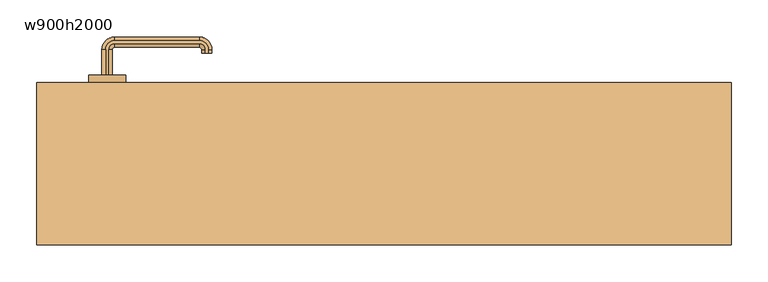
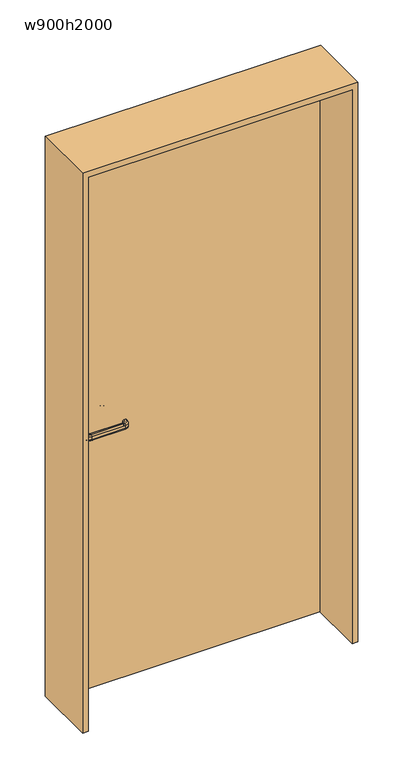
"""IFC4 building model written with IfcOpenShell, lengths in millimetres: door geometry, 片開き : w900h2000."""

from ifc_helpers import new_model, si_unit, point, frame, frame_2d, origin, origin_with_axes, place, context, project, spatial, polyline, circle_curve, ellipse_curve, trimmed, segment, composite_curve, outline, extrude, source, transform, mapped, element, save
from ifc_brep_helpers import plane_surface, cylinder_surface, revolved_surface, advanced_brep


def w900h2000_79a0ba88(model_context):
    return source(origin(), model_context, "Body", "SolidModel", [
        advanced_brep(
        [(-377.0, 120.0, 960.0), (-382.0, 120.0, 955.0), (-382.0, 120.0, 945.0477623), (-377.0, 120.0, 940.0477623), (-373.0, 120.0, 940.0477623), (-368.0, 120.0, 945.0477623), (-368.0, 120.0, 955.0), (-373.0, 120.0, 960.0), (-377.0, 155.0, 960.0), (-382.0, 155.0, 955.0), (-382.0, 155.0, 945.0477623), (-377.0, 155.0, 940.0477623), (-365.0, 167.0, 940.0477623), (-250.0, 167.0, 940.0477623), (-238.0, 155.0, 940.0477623), (-238.0, 150.0, 940.0477623), (-242.0, 150.0, 940.0477623), (-242.0, 155.0, 940.0477623), (-250.0, 163.0, 940.0477623), (-365.0, 163.0, 940.0477623), (-373.0, 155.0, 940.0477623), (-368.0, 155.0, 945.0477623), (-368.0, 155.0, 955.0), (-373.0, 155.0, 960.0), (-365.0, 163.0, 960.0), (-250.0, 163.0, 960.0), (-242.0, 155.0, 960.0), (-242.0, 150.0, 960.0), (-238.0, 150.0, 960.0), (-238.0, 155.0, 960.0), (-250.0, 167.0, 960.0), (-365.0, 167.0, 960.0), (-365.0, 172.0, 955.0), (-365.0, 172.0, 945.0477623), (-365.0, 158.0, 945.0477623), (-365.0, 158.0, 955.0), (-250.0, 172.0, 955.0), (-250.0, 172.0, 945.0477623), (-250.0, 158.0, 945.0477623), (-250.0, 158.0, 955.0), (-233.0, 155.0, 955.0), (-233.0, 155.0, 945.0477623), (-247.0, 155.0, 945.0477623), (-247.0, 155.0, 955.0), (-247.0, 150.0, 955.0), (-247.0, 150.0, 945.0477623), (-233.0, 150.0, 945.0477623), (-233.0, 150.0, 955.0)],
        [
            (0, 1, circle_curve(frame((-377.0, 120.0, 955.0), z_axis=(0.0, -1.0, 0.0), x_axis=(-1.0, 0.0, 0.0)), 5.0)),
            (1, 2),
            (2, 3, circle_curve(frame((-377.0, 120.0, 945.0477623), z_axis=(0.0, -1.0, 0.0), x_axis=(-1.0, 0.0, 0.0)), 5.0)),
            (3, 4),
            (4, 5, circle_curve(frame((-373.0, 120.0, 945.0477623), z_axis=(0.0, -1.0, 0.0), x_axis=(-1.0, 0.0, 0.0)), 5.0)),
            (5, 6),
            (6, 7, circle_curve(frame((-373.0, 120.0, 955.0), z_axis=(0.0, -1.0, 0.0), x_axis=(-1.0, 0.0, 0.0)), 5.0)),
            (7, 0),
            (0, 8),
            (8, 9, circle_curve(frame((-377.0, 155.0, 955.0), z_axis=(0.0, -1.0, 0.0), x_axis=(-1.0, 0.0, 0.0)), 5.0)),
            (9, 1),
            (9, 10),
            (10, 2),
            (10, 11, circle_curve(frame((-377.0, 155.0, 945.0477623), z_axis=(0.0, -1.0, 0.0), x_axis=(-1.0, 0.0, 0.0)), 5.0)),
            (11, 3),
            (11, 12, circle_curve(frame((-365.0, 155.0, 940.0477623), z_axis=(0.0, 0.0, -1.0), x_axis=(-1.0, 0.0, 0.0)), 12.0)),
            (12, 13),
            (13, 14, circle_curve(frame((-250.0, 155.0, 940.0477623), z_axis=(0.0, 0.0, -1.0), x_axis=(0.0, 1.0, 0.0)), 12.0)),
            (14, 15),
            (15, 16),
            (16, 17),
            (17, 18, circle_curve(frame((-250.0, 155.0, 940.0477623), z_axis=(0.0, 0.0, 1.0), x_axis=(0.0, 1.0, 0.0)), 8.0)),
            (18, 19),
            (19, 20, circle_curve(frame((-365.0, 155.0, 940.0477623), z_axis=(0.0, 0.0, 1.0), x_axis=(-1.0, 0.0, 0.0)), 8.0)),
            (20, 4),
            (20, 21, circle_curve(frame((-373.0, 155.0, 945.0477623), z_axis=(0.0, -1.0, 0.0), x_axis=(-1.0, 0.0, 0.0)), 5.0)),
            (21, 5),
            (21, 22),
            (22, 6),
            (22, 23, circle_curve(frame((-373.0, 155.0, 955.0), z_axis=(0.0, -1.0, 0.0), x_axis=(-1.0, 0.0, 0.0)), 5.0)),
            (23, 7),
            (23, 24, circle_curve(frame((-365.0, 155.0, 960.0), z_axis=(0.0, 0.0, -1.0), x_axis=(-1.0, 0.0, 0.0)), 8.0)),
            (24, 25),
            (25, 26, circle_curve(frame((-250.0, 155.0, 960.0), z_axis=(0.0, 0.0, -1.0), x_axis=(0.0, 1.0, 0.0)), 8.0)),
            (26, 27),
            (27, 28),
            (28, 29),
            (29, 30, circle_curve(frame((-250.0, 155.0, 960.0), z_axis=(0.0, 0.0, 1.0), x_axis=(0.0, 1.0, 0.0)), 12.0)),
            (30, 31),
            (31, 8, circle_curve(frame((-365.0, 155.0, 960.0), z_axis=(0.0, 0.0, 1.0), x_axis=(-1.0, 0.0, 0.0)), 12.0)),
            (32, 9, circle_curve(frame((-365.0, 155.0, 955.0), z_axis=(0.0, 0.0, 1.0), x_axis=(-1.0, 0.0, 0.0)), 17.0)),
            (31, 32, circle_curve(frame((-365.0, 167.0, 955.0), z_axis=(-1.0, 0.0, 0.0), x_axis=(0.0, 1.0, 0.0)), 5.0)),
            (33, 10, circle_curve(frame((-365.0, 155.0, 945.0477623), z_axis=(0.0, 0.0, 1.0), x_axis=(-1.0, 0.0, 0.0)), 17.0)),
            (32, 33),
            (33, 12, circle_curve(frame((-365.0, 167.0, 945.0477623), z_axis=(-1.0, 0.0, 0.0), x_axis=(0.0, 1.0, 0.0)), 5.0)),
            (34, 21, circle_curve(frame((-365.0, 155.0, 945.0477623), z_axis=(0.0, 0.0, 1.0), x_axis=(-1.0, 0.0, 0.0)), 3.0)),
            (19, 34, circle_curve(frame((-365.0, 163.0, 945.0477623), z_axis=(-1.0, 0.0, 0.0), x_axis=(0.0, 1.0, 0.0)), 5.0)),
            (35, 22, circle_curve(frame((-365.0, 155.0, 955.0), z_axis=(0.0, 0.0, 1.0), x_axis=(-1.0, 0.0, 0.0)), 3.0)),
            (34, 35),
            (35, 24, circle_curve(frame((-365.0, 163.0, 955.0), z_axis=(-1.0, 0.0, 0.0), x_axis=(0.0, 1.0, 0.0)), 5.0)),
            (30, 36, circle_curve(frame((-250.0, 167.0, 955.0), z_axis=(-1.0, 0.0, 0.0), x_axis=(0.0, 1.0, 0.0)), 5.0)),
            (36, 32),
            (36, 37),
            (37, 33),
            (37, 13, circle_curve(frame((-250.0, 167.0, 945.0477623), z_axis=(-1.0, 0.0, 0.0), x_axis=(0.0, 1.0, 0.0)), 5.0)),
            (18, 38, circle_curve(frame((-250.0, 163.0, 945.0477623), z_axis=(-1.0, 0.0, 0.0), x_axis=(0.0, 1.0, 0.0)), 5.0)),
            (38, 34),
            (38, 39),
            (39, 35),
            (39, 25, circle_curve(frame((-250.0, 163.0, 955.0), z_axis=(-1.0, 0.0, 0.0), x_axis=(0.0, 1.0, 0.0)), 5.0)),
            (40, 36, circle_curve(frame((-250.0, 155.0, 955.0), z_axis=(0.0, 0.0, 1.0), x_axis=(0.0, 1.0, 0.0)), 17.0)),
            (29, 40, circle_curve(frame((-238.0, 155.0, 955.0), z_axis=(0.0, 1.0, 0.0), x_axis=(1.0, 0.0, 0.0)), 5.0)),
            (41, 37, circle_curve(frame((-250.0, 155.0, 945.0477623), z_axis=(0.0, 0.0, 1.0), x_axis=(0.0, 1.0, 0.0)), 17.0)),
            (40, 41),
            (41, 14, circle_curve(frame((-238.0, 155.0, 945.0477623), z_axis=(0.0, 1.0, 0.0), x_axis=(1.0, 0.0, 0.0)), 5.0)),
            (42, 38, circle_curve(frame((-250.0, 155.0, 945.0477623), z_axis=(0.0, 0.0, 1.0), x_axis=(0.0, 1.0, 0.0)), 3.0)),
            (17, 42, circle_curve(frame((-242.0, 155.0, 945.0477623), z_axis=(0.0, 1.0, 0.0), x_axis=(1.0, 0.0, 0.0)), 5.0)),
            (43, 39, circle_curve(frame((-250.0, 155.0, 955.0), z_axis=(0.0, 0.0, 1.0), x_axis=(0.0, 1.0, 0.0)), 3.0)),
            (42, 43),
            (43, 26, circle_curve(frame((-242.0, 155.0, 955.0), z_axis=(0.0, 1.0, 0.0), x_axis=(1.0, 0.0, 0.0)), 5.0)),
            (27, 44, circle_curve(frame((-242.0, 150.0, 955.0), z_axis=(0.0, -1.0, 0.0), x_axis=(1.0, 0.0, 0.0)), 5.0)),
            (44, 45),
            (45, 16, circle_curve(frame((-242.0, 150.0, 945.0477623), z_axis=(0.0, -1.0, 0.0), x_axis=(1.0, 0.0, 0.0)), 5.0)),
            (15, 46, circle_curve(frame((-238.0, 150.0, 945.0477623), z_axis=(0.0, -1.0, 0.0), x_axis=(1.0, 0.0, 0.0)), 5.0)),
            (46, 47),
            (47, 28, circle_curve(frame((-238.0, 150.0, 955.0), z_axis=(0.0, -1.0, 0.0), x_axis=(1.0, 0.0, 0.0)), 5.0)),
            (47, 40),
            (46, 41),
            (45, 42),
            (44, 43),
        ],
        [
            plane_surface(frame((-385.198039, 120.0, 950.0), z_axis=(0.0, -1.0, 0.0), x_axis=(0.0, 0.0, 1.0))),
            cylinder_surface(frame((-377.0, 120.0, 955.0), z_axis=(0.0, -1.0, 0.0), x_axis=(-1.0, 0.0, 0.0)), 5.0),
            plane_surface(frame((-382.0, 120.0, 955.0), z_axis=(-1.0, 0.0, 0.0), x_axis=(0.0, 1.0, 0.0))),
            cylinder_surface(frame((-377.0, 120.0, 945.0477623), z_axis=(0.0, -1.0, 0.0), x_axis=(-1.0, 0.0, 0.0)), 5.0),
            plane_surface(frame((-377.0, 120.0, 940.0477623), z_axis=(0.0, 0.0, -1.0), x_axis=(0.0, 1.0, 0.0))),
            cylinder_surface(frame((-373.0, 120.0, 945.0477623), z_axis=(0.0, -1.0, 0.0), x_axis=(-1.0, 0.0, 0.0)), 5.0),
            plane_surface(frame((-368.0, 120.0, 945.0477623), z_axis=(1.0, 0.0, 0.0), x_axis=(0.0, 1.0, 0.0))),
            cylinder_surface(frame((-373.0, 120.0, 955.0), z_axis=(0.0, -1.0, 0.0), x_axis=(-1.0, 0.0, 0.0)), 5.0),
            plane_surface(frame((-373.0, 120.0, 960.0), z_axis=(0.0, 0.0, 1.0), x_axis=(0.0, 1.0, 0.0))),
            revolved_surface(trimmed(ellipse_curve(frame((-377.0, 155.0, 955.0), z_axis=(0.0, -1.0, 0.0), x_axis=(-1.0, 0.0, 0.0)), 5.0, 5.0), [point((-377.0, 155.0, 960.0))], [point((-382.0, 155.0, 955.0))], True, "CARTESIAN"), (-365.0, 155.0, 950.0), (0.0, 0.0, -1.0)),
            cylinder_surface(frame((-365.0, 155.0, 950.0), z_axis=(0.0, 0.0, -1.0), x_axis=(-1.0, 0.0, 0.0)), 17.0),
            revolved_surface(trimmed(ellipse_curve(frame((-377.0, 155.0, 945.0477623), z_axis=(0.0, -1.0, 0.0), x_axis=(-1.0, 0.0, 0.0)), 5.0, 5.0), [point((-382.0, 155.0, 945.0477623))], [point((-377.0, 155.0, 940.0477623))], True, "CARTESIAN"), (-365.0, 155.0, 950.0), (0.0, 0.0, -1.0)),
            revolved_surface(trimmed(ellipse_curve(frame((-373.0, 155.0, 945.0477623), z_axis=(0.0, -1.0, 0.0), x_axis=(-1.0, 0.0, 0.0)), 5.0, 5.0), [point((-373.0, 155.0, 940.0477623))], [point((-368.0, 155.0, 945.0477623))], True, "CARTESIAN"), (-365.0, 155.0, 950.0), (0.0, 0.0, -1.0)),
            revolved_surface(polyline([(-368.0, 155.0, 945.0477623), (-368.0, 155.0, 955.0)]), (-365.0, 155.0, 950.0), (0.0, 0.0, -1.0)),
            revolved_surface(trimmed(ellipse_curve(frame((-373.0, 155.0, 955.0), z_axis=(0.0, -1.0, 0.0), x_axis=(-1.0, 0.0, 0.0)), 5.0, 5.0), [point((-368.0, 155.0, 955.0))], [point((-373.0, 155.0, 960.0))], True, "CARTESIAN"), (-365.0, 155.0, 950.0), (0.0, 0.0, -1.0)),
            cylinder_surface(frame((-365.0, 167.0, 955.0), z_axis=(-1.0, 0.0, 0.0), x_axis=(0.0, 1.0, 0.0)), 5.0),
            plane_surface(frame((-365.0, 172.0, 955.0), z_axis=(0.0, 1.0, 0.0), x_axis=(1.0, 0.0, 0.0))),
            cylinder_surface(frame((-365.0, 167.0, 945.0477623), z_axis=(-1.0, 0.0, 0.0), x_axis=(0.0, 1.0, 0.0)), 5.0),
            cylinder_surface(frame((-365.0, 163.0, 945.0477623), z_axis=(-1.0, 0.0, 0.0), x_axis=(0.0, 1.0, 0.0)), 5.0),
            plane_surface(frame((-365.0, 158.0, 945.0477623), z_axis=(0.0, -1.0, 0.0), x_axis=(1.0, 0.0, 0.0))),
            cylinder_surface(frame((-365.0, 163.0, 955.0), z_axis=(-1.0, 0.0, 0.0), x_axis=(0.0, 1.0, 0.0)), 5.0),
            revolved_surface(trimmed(ellipse_curve(frame((-250.0, 167.0, 955.0), z_axis=(-1.0, 0.0, 0.0), x_axis=(0.0, 1.0, 0.0)), 5.0, 5.0), [point((-250.0, 167.0, 960.0))], [point((-250.0, 172.0, 955.0))], True, "CARTESIAN"), (-250.0, 155.0, 950.0), (0.0, 0.0, -1.0)),
            cylinder_surface(frame((-250.0, 155.0, 950.0), z_axis=(0.0, 0.0, -1.0), x_axis=(0.0, 1.0, 0.0)), 17.0),
            revolved_surface(trimmed(ellipse_curve(frame((-250.0, 167.0, 945.0477623), z_axis=(-1.0, 0.0, 0.0), x_axis=(0.0, 1.0, 0.0)), 5.0, 5.0), [point((-250.0, 172.0, 945.0477623))], [point((-250.0, 167.0, 940.0477623))], True, "CARTESIAN"), (-250.0, 155.0, 950.0), (0.0, 0.0, -1.0)),
            revolved_surface(trimmed(ellipse_curve(frame((-250.0, 163.0, 945.0477623), z_axis=(-1.0, 0.0, 0.0), x_axis=(0.0, 1.0, 0.0)), 5.0, 5.0), [point((-250.0, 163.0, 940.0477623))], [point((-250.0, 158.0, 945.0477623))], True, "CARTESIAN"), (-250.0, 155.0, 950.0), (0.0, 0.0, -1.0)),
            revolved_surface(polyline([(-250.0, 158.0, 945.0477623), (-250.0, 158.0, 955.0)]), (-250.0, 155.0, 950.0), (0.0, 0.0, -1.0)),
            revolved_surface(trimmed(ellipse_curve(frame((-250.0, 163.0, 955.0), z_axis=(-1.0, 0.0, 0.0), x_axis=(0.0, 1.0, 0.0)), 5.0, 5.0), [point((-250.0, 158.0, 955.0))], [point((-250.0, 163.0, 960.0))], True, "CARTESIAN"), (-250.0, 155.0, 950.0), (0.0, 0.0, -1.0)),
            plane_surface(frame((-250.198039, 150.0, 950.0), z_axis=(0.0, -1.0, 0.0), x_axis=(0.0, 0.0, -1.0))),
            cylinder_surface(frame((-238.0, 155.0, 955.0), z_axis=(0.0, 1.0, 0.0), x_axis=(1.0, 0.0, 0.0)), 5.0),
            plane_surface(frame((-233.0, 155.0, 955.0), z_axis=(1.0, 0.0, 0.0), x_axis=(0.0, -1.0, 0.0))),
            cylinder_surface(frame((-238.0, 155.0, 945.0477623), z_axis=(0.0, 1.0, 0.0), x_axis=(1.0, 0.0, 0.0)), 5.0),
            cylinder_surface(frame((-242.0, 155.0, 945.0477623), z_axis=(0.0, 1.0, 0.0), x_axis=(1.0, 0.0, 0.0)), 5.0),
            plane_surface(frame((-247.0, 155.0, 945.0477623), z_axis=(-1.0, 0.0, 0.0), x_axis=(0.0, -1.0, 0.0))),
            cylinder_surface(frame((-242.0, 155.0, 955.0), z_axis=(0.0, 1.0, 0.0), x_axis=(1.0, 0.0, 0.0)), 5.0),
        ],
        [
            (0, [[1, 2, 3, 4, 5, 6, 7, 8]]),
            (1, [[-1, 9, 10, 11]]),
            (2, [[-2, -11, 12, 13]]),
            (3, [[-3, -13, 14, 15]]),
            (4, [[-4, -15, 16, 17, 18, 19, 20, 21, 22, 23, 24, 25]]),
            (5, [[-5, -25, 26, 27]]),
            (6, [[-6, -27, 28, 29]]),
            (7, [[-7, -29, 30, 31]]),
            (8, [[-8, -31, 32, 33, 34, 35, 36, 37, 38, 39, 40, -9]]),
            (9, [[41, -10, -40, 42]]),
            (10, [[43, -12, -41, 44]]),
            (11, [[-16, -14, -43, 45]]),
            (12, [[46, -26, -24, 47]]),
            (13, [[48, -28, -46, 49]]),
            (14, [[-32, -30, -48, 50]]),
            (15, [[-42, -39, 51, 52]]),
            (16, [[-44, -52, 53, 54]]),
            (17, [[-45, -54, 55, -17]]),
            (18, [[-47, -23, 56, 57]]),
            (19, [[-49, -57, 58, 59]]),
            (20, [[-50, -59, 60, -33]]),
            (21, [[61, -51, -38, 62]]),
            (22, [[63, -53, -61, 64]]),
            (23, [[-18, -55, -63, 65]]),
            (24, [[66, -56, -22, 67]]),
            (25, [[68, -58, -66, 69]]),
            (26, [[-34, -60, -68, 70]]),
            (27, [[-36, 71, 72, 73, -20, 74, 75, 76]]),
            (28, [[-62, -37, -76, 77]]),
            (29, [[-64, -77, -75, 78]]),
            (30, [[-65, -78, -74, -19]]),
            (31, [[-67, -21, -73, 79]]),
            (32, [[-69, -79, -72, 80]]),
            (33, [[-70, -80, -71, -35]]),
        ],
    ),
        advanced_brep(
        [(-373.0, 70.0, 940.0), (-377.0, 70.0, 940.0), (-382.0, 70.0, 945.0), (-382.0, 70.0, 955.0), (-377.0, 70.0, 960.0), (-373.0, 70.0, 960.0), (-368.0, 70.0, 955.0), (-368.0, 70.0, 945.0), (-373.0, 35.0, 940.0), (-365.0, 27.0, 940.0), (-250.0, 27.0, 940.0), (-242.0, 35.0, 940.0), (-242.0, 40.0, 940.0), (-238.0, 40.0, 940.0), (-238.0, 35.0, 940.0), (-250.0, 23.0, 940.0), (-365.0, 23.0, 940.0), (-377.0, 35.0, 940.0), (-382.0, 35.0, 945.0), (-382.0, 35.0, 955.0), (-377.0, 35.0, 960.0), (-365.0, 23.0, 960.0), (-250.0, 23.0, 960.0), (-238.0, 35.0, 960.0), (-238.0, 40.0, 960.0), (-242.0, 40.0, 960.0), (-242.0, 35.0, 960.0), (-250.0, 27.0, 960.0), (-365.0, 27.0, 960.0), (-373.0, 35.0, 960.0), (-368.0, 35.0, 955.0), (-368.0, 35.0, 945.0), (-365.0, 18.0, 945.0), (-365.0, 18.0, 955.0), (-365.0, 32.0, 955.0), (-365.0, 32.0, 945.0), (-250.0, 18.0, 945.0), (-250.0, 18.0, 955.0), (-250.0, 32.0, 955.0), (-250.0, 32.0, 945.0), (-233.0, 35.0, 945.0), (-233.0, 35.0, 955.0), (-247.0, 35.0, 955.0), (-247.0, 35.0, 945.0), (-247.0, 40.0, 945.0), (-247.0, 40.0, 955.0), (-233.0, 40.0, 955.0), (-233.0, 40.0, 945.0)],
        [
            (0, 1),
            (1, 2, circle_curve(frame((-377.0, 70.0, 945.0), z_axis=(0.0, 1.0, 0.0), x_axis=(1.0, 0.0, 0.0)), 5.0)),
            (2, 3),
            (3, 4, circle_curve(frame((-377.0, 70.0, 955.0), z_axis=(0.0, 1.0, 0.0), x_axis=(1.0, 0.0, 0.0)), 5.0)),
            (4, 5),
            (5, 6, circle_curve(frame((-373.0, 70.0, 955.0), z_axis=(0.0, 1.0, 0.0), x_axis=(1.0, 0.0, 0.0)), 5.0)),
            (6, 7),
            (7, 0, circle_curve(frame((-373.0, 70.0, 945.0), z_axis=(0.0, 1.0, 0.0), x_axis=(1.0, 0.0, 0.0)), 5.0)),
            (0, 8),
            (8, 9, circle_curve(frame((-365.0, 35.0, 940.0), z_axis=(0.0, 0.0, 1.0), x_axis=(-1.0, 0.0, 0.0)), 8.0)),
            (9, 10),
            (10, 11, circle_curve(frame((-250.0, 35.0, 940.0), z_axis=(0.0, 0.0, 1.0), x_axis=(0.0, -1.0, 0.0)), 8.0)),
            (11, 12),
            (12, 13),
            (13, 14),
            (14, 15, circle_curve(frame((-250.0, 35.0, 940.0), z_axis=(0.0, 0.0, -1.0), x_axis=(0.0, -1.0, 0.0)), 12.0)),
            (15, 16),
            (16, 17, circle_curve(frame((-365.0, 35.0, 940.0), z_axis=(0.0, 0.0, -1.0), x_axis=(-1.0, 0.0, 0.0)), 12.0)),
            (17, 1),
            (17, 18, circle_curve(frame((-377.0, 35.0, 945.0), z_axis=(0.0, 1.0, 0.0), x_axis=(1.0, 0.0, 0.0)), 5.0)),
            (18, 2),
            (18, 19),
            (19, 3),
            (19, 20, circle_curve(frame((-377.0, 35.0, 955.0), z_axis=(0.0, 1.0, 0.0), x_axis=(1.0, 0.0, 0.0)), 5.0)),
            (20, 4),
            (20, 21, circle_curve(frame((-365.0, 35.0, 960.0), z_axis=(0.0, 0.0, 1.0), x_axis=(-1.0, 0.0, 0.0)), 12.0)),
            (21, 22),
            (22, 23, circle_curve(frame((-250.0, 35.0, 960.0), z_axis=(0.0, 0.0, 1.0), x_axis=(0.0, -1.0, 0.0)), 12.0)),
            (23, 24),
            (24, 25),
            (25, 26),
            (26, 27, circle_curve(frame((-250.0, 35.0, 960.0), z_axis=(0.0, 0.0, -1.0), x_axis=(0.0, -1.0, 0.0)), 8.0)),
            (27, 28),
            (28, 29, circle_curve(frame((-365.0, 35.0, 960.0), z_axis=(0.0, 0.0, -1.0), x_axis=(-1.0, 0.0, 0.0)), 8.0)),
            (29, 5),
            (29, 30, circle_curve(frame((-373.0, 35.0, 955.0), z_axis=(0.0, 1.0, 0.0), x_axis=(1.0, 0.0, 0.0)), 5.0)),
            (30, 6),
            (30, 31),
            (31, 7),
            (31, 8, circle_curve(frame((-373.0, 35.0, 945.0), z_axis=(0.0, 1.0, 0.0), x_axis=(1.0, 0.0, 0.0)), 5.0)),
            (32, 18, circle_curve(frame((-365.0, 35.0, 945.0), z_axis=(0.0, 0.0, -1.0), x_axis=(-1.0, 0.0, 0.0)), 17.0)),
            (16, 32, circle_curve(frame((-365.0, 23.0, 945.0), z_axis=(-1.0, 0.0, 0.0), x_axis=(0.0, 1.0, 0.0)), 5.0)),
            (33, 19, circle_curve(frame((-365.0, 35.0, 955.0), z_axis=(0.0, 0.0, -1.0), x_axis=(-1.0, 0.0, 0.0)), 17.0)),
            (32, 33),
            (33, 21, circle_curve(frame((-365.0, 23.0, 955.0), z_axis=(-1.0, 0.0, 0.0), x_axis=(0.0, 1.0, 0.0)), 5.0)),
            (34, 30, circle_curve(frame((-365.0, 35.0, 955.0), z_axis=(0.0, 0.0, -1.0), x_axis=(-1.0, 0.0, 0.0)), 3.0)),
            (28, 34, circle_curve(frame((-365.0, 27.0, 955.0), z_axis=(-1.0, 0.0, 0.0), x_axis=(0.0, 1.0, 0.0)), 5.0)),
            (35, 31, circle_curve(frame((-365.0, 35.0, 945.0), z_axis=(0.0, 0.0, -1.0), x_axis=(-1.0, 0.0, 0.0)), 3.0)),
            (34, 35),
            (35, 9, circle_curve(frame((-365.0, 27.0, 945.0), z_axis=(-1.0, 0.0, 0.0), x_axis=(0.0, 1.0, 0.0)), 5.0)),
            (15, 36, circle_curve(frame((-250.0, 23.0, 945.0), z_axis=(-1.0, 0.0, 0.0), x_axis=(0.0, 1.0, 0.0)), 5.0)),
            (36, 32),
            (36, 37),
            (37, 33),
            (37, 22, circle_curve(frame((-250.0, 23.0, 955.0), z_axis=(-1.0, 0.0, 0.0), x_axis=(0.0, 1.0, 0.0)), 5.0)),
            (27, 38, circle_curve(frame((-250.0, 27.0, 955.0), z_axis=(-1.0, 0.0, 0.0), x_axis=(0.0, 1.0, 0.0)), 5.0)),
            (38, 34),
            (38, 39),
            (39, 35),
            (39, 10, circle_curve(frame((-250.0, 27.0, 945.0), z_axis=(-1.0, 0.0, 0.0), x_axis=(0.0, 1.0, 0.0)), 5.0)),
            (40, 36, circle_curve(frame((-250.0, 35.0, 945.0), z_axis=(0.0, 0.0, -1.0), x_axis=(0.0, -1.0, 0.0)), 17.0)),
            (14, 40, circle_curve(frame((-238.0, 35.0, 945.0), z_axis=(0.0, -1.0, 0.0), x_axis=(-1.0, 0.0, 0.0)), 5.0)),
            (41, 37, circle_curve(frame((-250.0, 35.0, 955.0), z_axis=(0.0, 0.0, -1.0), x_axis=(0.0, -1.0, 0.0)), 17.0)),
            (40, 41),
            (41, 23, circle_curve(frame((-238.0, 35.0, 955.0), z_axis=(0.0, -1.0, 0.0), x_axis=(-1.0, 0.0, 0.0)), 5.0)),
            (42, 38, circle_curve(frame((-250.0, 35.0, 955.0), z_axis=(0.0, 0.0, -1.0), x_axis=(0.0, -1.0, 0.0)), 3.0)),
            (26, 42, circle_curve(frame((-242.0, 35.0, 955.0), z_axis=(0.0, -1.0, 0.0), x_axis=(-1.0, 0.0, 0.0)), 5.0)),
            (43, 39, circle_curve(frame((-250.0, 35.0, 945.0), z_axis=(0.0, 0.0, -1.0), x_axis=(0.0, -1.0, 0.0)), 3.0)),
            (42, 43),
            (43, 11, circle_curve(frame((-242.0, 35.0, 945.0), z_axis=(0.0, -1.0, 0.0), x_axis=(-1.0, 0.0, 0.0)), 5.0)),
            (12, 44, circle_curve(frame((-242.0, 40.0, 945.0), z_axis=(0.0, 1.0, 0.0), x_axis=(-1.0, 0.0, 0.0)), 5.0)),
            (44, 45),
            (45, 25, circle_curve(frame((-242.0, 40.0, 955.0), z_axis=(0.0, 1.0, 0.0), x_axis=(-1.0, 0.0, 0.0)), 5.0)),
            (24, 46, circle_curve(frame((-238.0, 40.0, 955.0), z_axis=(0.0, 1.0, 0.0), x_axis=(-1.0, 0.0, 0.0)), 5.0)),
            (46, 47),
            (47, 13, circle_curve(frame((-238.0, 40.0, 945.0), z_axis=(0.0, 1.0, 0.0), x_axis=(-1.0, 0.0, 0.0)), 5.0)),
            (47, 40),
            (46, 41),
            (45, 42),
            (44, 43),
        ],
        [
            plane_surface(frame((-385.198039, 70.0, 950.0), z_axis=(0.0, 1.0, 0.0), x_axis=(0.0, 0.0, -1.0))),
            plane_surface(frame((-373.0, 70.0, 940.0), z_axis=(0.0, 0.0, -1.0), x_axis=(0.0, -1.0, 0.0))),
            cylinder_surface(frame((-377.0, 70.0, 945.0), z_axis=(0.0, 1.0, 0.0), x_axis=(1.0, 0.0, 0.0)), 5.0),
            plane_surface(frame((-382.0, 70.0, 945.0), z_axis=(-1.0, 0.0, 0.0), x_axis=(0.0, -1.0, 0.0))),
            cylinder_surface(frame((-377.0, 70.0, 955.0), z_axis=(0.0, 1.0, 0.0), x_axis=(1.0, 0.0, 0.0)), 5.0),
            plane_surface(frame((-377.0, 70.0, 960.0), z_axis=(0.0, 0.0, 1.0), x_axis=(0.0, -1.0, 0.0))),
            cylinder_surface(frame((-373.0, 70.0, 955.0), z_axis=(0.0, 1.0, 0.0), x_axis=(1.0, 0.0, 0.0)), 5.0),
            plane_surface(frame((-368.0, 70.0, 955.0), z_axis=(1.0, 0.0, 0.0), x_axis=(0.0, -1.0, 0.0))),
            cylinder_surface(frame((-373.0, 70.0, 945.0), z_axis=(0.0, 1.0, 0.0), x_axis=(1.0, 0.0, 0.0)), 5.0),
            revolved_surface(trimmed(ellipse_curve(frame((-377.0, 35.0, 945.0), z_axis=(0.0, 1.0, 0.0), x_axis=(1.0, 0.0, 0.0)), 5.0, 5.0), [point((-377.0, 35.0, 940.0))], [point((-382.0, 35.0, 945.0))], True, "CARTESIAN"), (-365.0, 35.0, 950.0), (0.0, 0.0, 1.0)),
            cylinder_surface(frame((-365.0, 35.0, 950.0), z_axis=(0.0, 0.0, 1.0), x_axis=(-1.0, 0.0, 0.0)), 17.0),
            revolved_surface(trimmed(ellipse_curve(frame((-377.0, 35.0, 955.0), z_axis=(0.0, 1.0, 0.0), x_axis=(1.0, 0.0, 0.0)), 5.0, 5.0), [point((-382.0, 35.0, 955.0))], [point((-377.0, 35.0, 960.0))], True, "CARTESIAN"), (-365.0, 35.0, 950.0), (0.0, 0.0, 1.0)),
            revolved_surface(trimmed(ellipse_curve(frame((-373.0, 35.0, 955.0), z_axis=(0.0, 1.0, 0.0), x_axis=(1.0, 0.0, 0.0)), 5.0, 5.0), [point((-373.0, 35.0, 960.0))], [point((-368.0, 35.0, 955.0))], True, "CARTESIAN"), (-365.0, 35.0, 950.0), (0.0, 0.0, 1.0)),
            revolved_surface(polyline([(-368.0, 35.0, 955.0), (-368.0, 35.0, 945.0)]), (-365.0, 35.0, 950.0), (0.0, 0.0, 1.0)),
            revolved_surface(trimmed(ellipse_curve(frame((-373.0, 35.0, 945.0), z_axis=(0.0, 1.0, 0.0), x_axis=(1.0, 0.0, 0.0)), 5.0, 5.0), [point((-368.0, 35.0, 945.0))], [point((-373.0, 35.0, 940.0))], True, "CARTESIAN"), (-365.0, 35.0, 950.0), (0.0, 0.0, 1.0)),
            cylinder_surface(frame((-365.0, 23.0, 945.0), z_axis=(-1.0, 0.0, 0.0), x_axis=(0.0, 1.0, 0.0)), 5.0),
            plane_surface(frame((-365.0, 18.0, 945.0), z_axis=(0.0, -1.0, 0.0), x_axis=(1.0, 0.0, 0.0))),
            cylinder_surface(frame((-365.0, 23.0, 955.0), z_axis=(-1.0, 0.0, 0.0), x_axis=(0.0, 1.0, 0.0)), 5.0),
            cylinder_surface(frame((-365.0, 27.0, 955.0), z_axis=(-1.0, 0.0, 0.0), x_axis=(0.0, 1.0, 0.0)), 5.0),
            plane_surface(frame((-365.0, 32.0, 955.0), z_axis=(0.0, 1.0, 0.0), x_axis=(1.0, 0.0, 0.0))),
            cylinder_surface(frame((-365.0, 27.0, 945.0), z_axis=(-1.0, 0.0, 0.0), x_axis=(0.0, 1.0, 0.0)), 5.0),
            revolved_surface(trimmed(ellipse_curve(frame((-250.0, 23.0, 945.0), z_axis=(-1.0, 0.0, 0.0), x_axis=(0.0, 1.0, 0.0)), 5.0, 5.0), [point((-250.0, 23.0, 940.0))], [point((-250.0, 18.0, 945.0))], True, "CARTESIAN"), (-250.0, 35.0, 950.0), (0.0, 0.0, 1.0)),
            cylinder_surface(frame((-250.0, 35.0, 950.0), z_axis=(0.0, 0.0, 1.0), x_axis=(0.0, -1.0, 0.0)), 17.0),
            revolved_surface(trimmed(ellipse_curve(frame((-250.0, 23.0, 955.0), z_axis=(-1.0, 0.0, 0.0), x_axis=(0.0, 1.0, 0.0)), 5.0, 5.0), [point((-250.0, 18.0, 955.0))], [point((-250.0, 23.0, 960.0))], True, "CARTESIAN"), (-250.0, 35.0, 950.0), (0.0, 0.0, 1.0)),
            revolved_surface(trimmed(ellipse_curve(frame((-250.0, 27.0, 955.0), z_axis=(-1.0, 0.0, 0.0), x_axis=(0.0, 1.0, 0.0)), 5.0, 5.0), [point((-250.0, 27.0, 960.0))], [point((-250.0, 32.0, 955.0))], True, "CARTESIAN"), (-250.0, 35.0, 950.0), (0.0, 0.0, 1.0)),
            revolved_surface(polyline([(-250.0, 32.0, 955.0), (-250.0, 32.0, 945.0)]), (-250.0, 35.0, 950.0), (0.0, 0.0, 1.0)),
            revolved_surface(trimmed(ellipse_curve(frame((-250.0, 27.0, 945.0), z_axis=(-1.0, 0.0, 0.0), x_axis=(0.0, 1.0, 0.0)), 5.0, 5.0), [point((-250.0, 32.0, 945.0))], [point((-250.0, 27.0, 940.0))], True, "CARTESIAN"), (-250.0, 35.0, 950.0), (0.0, 0.0, 1.0)),
            plane_surface(frame((-250.198039, 40.0, 950.0), z_axis=(0.0, 1.0, 0.0), x_axis=(0.0, 0.0, 1.0))),
            cylinder_surface(frame((-238.0, 35.0, 945.0), z_axis=(0.0, -1.0, 0.0), x_axis=(-1.0, 0.0, 0.0)), 5.0),
            plane_surface(frame((-233.0, 35.0, 945.0), z_axis=(1.0, 0.0, 0.0), x_axis=(0.0, 1.0, 0.0))),
            cylinder_surface(frame((-238.0, 35.0, 955.0), z_axis=(0.0, -1.0, 0.0), x_axis=(-1.0, 0.0, 0.0)), 5.0),
            cylinder_surface(frame((-242.0, 35.0, 955.0), z_axis=(0.0, -1.0, 0.0), x_axis=(-1.0, 0.0, 0.0)), 5.0),
            plane_surface(frame((-247.0, 35.0, 955.0), z_axis=(-1.0, 0.0, 0.0), x_axis=(0.0, 1.0, 0.0))),
            cylinder_surface(frame((-242.0, 35.0, 945.0), z_axis=(0.0, -1.0, 0.0), x_axis=(-1.0, 0.0, 0.0)), 5.0),
        ],
        [
            (0, [[1, 2, 3, 4, 5, 6, 7, 8]]),
            (1, [[-1, 9, 10, 11, 12, 13, 14, 15, 16, 17, 18, 19]]),
            (2, [[-2, -19, 20, 21]]),
            (3, [[-3, -21, 22, 23]]),
            (4, [[-4, -23, 24, 25]]),
            (5, [[-5, -25, 26, 27, 28, 29, 30, 31, 32, 33, 34, 35]]),
            (6, [[-6, -35, 36, 37]]),
            (7, [[-7, -37, 38, 39]]),
            (8, [[-8, -39, 40, -9]]),
            (9, [[41, -20, -18, 42]]),
            (10, [[43, -22, -41, 44]]),
            (11, [[-26, -24, -43, 45]]),
            (12, [[46, -36, -34, 47]]),
            (13, [[48, -38, -46, 49]]),
            (14, [[-10, -40, -48, 50]]),
            (15, [[-42, -17, 51, 52]]),
            (16, [[-44, -52, 53, 54]]),
            (17, [[-45, -54, 55, -27]]),
            (18, [[-47, -33, 56, 57]]),
            (19, [[-49, -57, 58, 59]]),
            (20, [[-50, -59, 60, -11]]),
            (21, [[61, -51, -16, 62]]),
            (22, [[63, -53, -61, 64]]),
            (23, [[-28, -55, -63, 65]]),
            (24, [[66, -56, -32, 67]]),
            (25, [[68, -58, -66, 69]]),
            (26, [[-12, -60, -68, 70]]),
            (27, [[71, 72, 73, -30, 74, 75, 76, -14]]),
            (28, [[-62, -15, -76, 77]]),
            (29, [[-64, -77, -75, 78]]),
            (30, [[-65, -78, -74, -29]]),
            (31, [[-67, -31, -73, 79]]),
            (32, [[-69, -79, -72, 80]]),
            (33, [[-70, -80, -71, -13]]),
        ],
    ),
        extrude(outline(composite_curve([segment(trimmed(circle_curve(frame_2d((950.0, -375.0)), 25.0), [point((950.0, -400.0))], [point((950.0, -350.0))], False, "CARTESIAN"), True, "CONTINUOUS"), segment(trimmed(circle_curve(frame_2d((950.0, -375.0)), 25.0), [point((950.0, -350.0))], [point((950.0, -400.0))], False, "CARTESIAN"), True, "CONTINUOUS")], self_intersect=False)), frame((0.0, 110.0, 0.0), z_axis=(0.0, 1.0, 0.0), x_axis=(0.0, 0.0, 1.0)), (0.0, 0.0, 1.0), 10.0),
        extrude(outline(composite_curve([segment(trimmed(circle_curve(frame_2d((950.0, -375.0)), 25.0), [point((950.0, -400.0))], [point((950.0, -350.0))], False, "CARTESIAN"), True, "CONTINUOUS"), segment(trimmed(circle_curve(frame_2d((950.0, -375.0)), 25.0), [point((950.0, -350.0))], [point((950.0, -400.0))], False, "CARTESIAN"), True, "CONTINUOUS")], self_intersect=False)), frame((0.0, 70.0, 0.0), z_axis=(0.0, 1.0, 0.0), x_axis=(0.0, 0.0, 1.0)), (0.0, 0.0, 1.0), 10.0),
        extrude(outline(polyline([(2020.0, -470.0), (0.0, -470.0), (0.0, -450.0), (2000.0, -450.0), (2000.0, 450.0), (0.0, 450.0), (0.0, 470.0), (2020.0, 470.0), (2020.0, -470.0)])), frame((0.0, -110.0, 0.0), z_axis=(0.0, 1.0, 0.0), x_axis=(0.0, 0.0, 1.0)), (0.0, 0.0, 1.0), 220.0),
        extrude(outline(polyline([(450.0, 80.0), (-450.0, 80.0), (-450.0, 110.0), (450.0, 110.0), (450.0, 80.0)])), origin_with_axes(), (0.0, 0.0, 1.0), 2000.0),
    ])


if __name__ == "__main__":
    model = new_model("IFC4")
    model_context = context("Model", 3, world=origin())
    ifc_project = project(units=[si_unit("LENGTHUNIT", "METRE", prefix="MILLI")], contexts=[model_context])
    site = spatial("IfcSite", under=ifc_project)
    building = spatial("IfcBuilding", under=site)
    placement = place(None, origin())
    w900h2000_shape = w900h2000_79a0ba88(model_context)
    element("IfcDoor", 1, ObjectType="片開き : w900h2000", at=placement, inside=building, context=model_context, shape_type="MappedRepresentation", body=[
        mapped(w900h2000_shape, transform((0.0, 0.0, 0.0), x_axis=(1.0, 0.0, 0.0), y_axis=(0.0, 1.0, 0.0), z_axis=(0.0, 0.0, 1.0))),
    ])
    save(model, "model.ifc")

# Revit data of these elements
# Type "片開き : w900h2000"
#   Type Mark = "23"
#   Operation = "片側開き戸右"
#   Keynote = "08110.P2"
#   Analytic Construction = "メタル"
#   Thermal Resistance (R) = 0.270117 (m²·K)/W
#   高さ(中心) = 1000 mm
#   Height = 2000 mm
#   Thickness = 30 mm
#   Heat Transfer Coefficient (U) = 3.7021 W/(m²·K)
#   ドア枠見附 = 20 mm
#   Width = 900 mm
#   取手取付け高さ = 950 mm
#   ドア枠ちり = 10 mm
#   Define Thermal Properties by = 1
#   ドア枠 [instance default] = 塗装ホワイト
#   ドア把手 [instance default] = メタル-ステンレス
#   ドア [instance default] = 塗装ホワイト
#   Visual Light Transmittance = 0
#   Solar Heat Gain Coefficient = 0
#   Function = (empty or 0)
#   Wall Closure = (empty or 0)
# Element 1 (IfcDoor, "片開き : w900h2000")
#   Materials on its faces: "メタル-ステンレス", "塗装ホワイト"
# Materials
#   "塗装ホワイト": class "ペイント", colour RGB 249 249 249, transparency 0
#   "メタル-ステンレス": class "メタル", colour RGB 247 247 247, transparency 0
